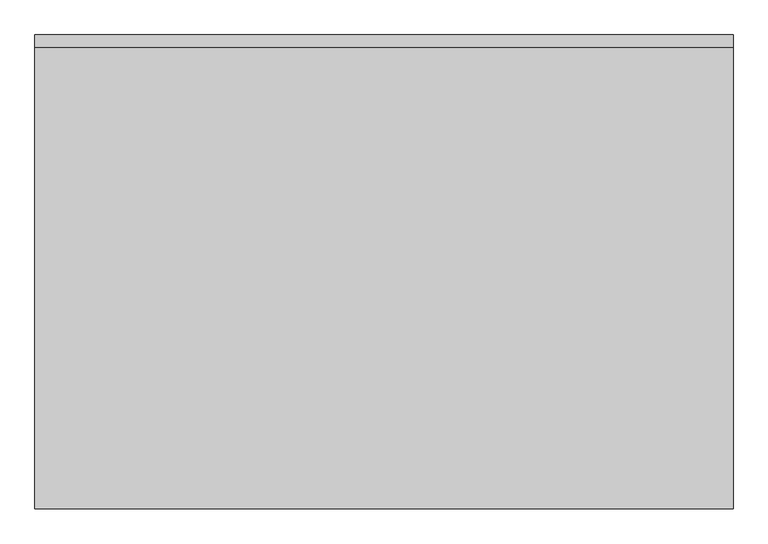
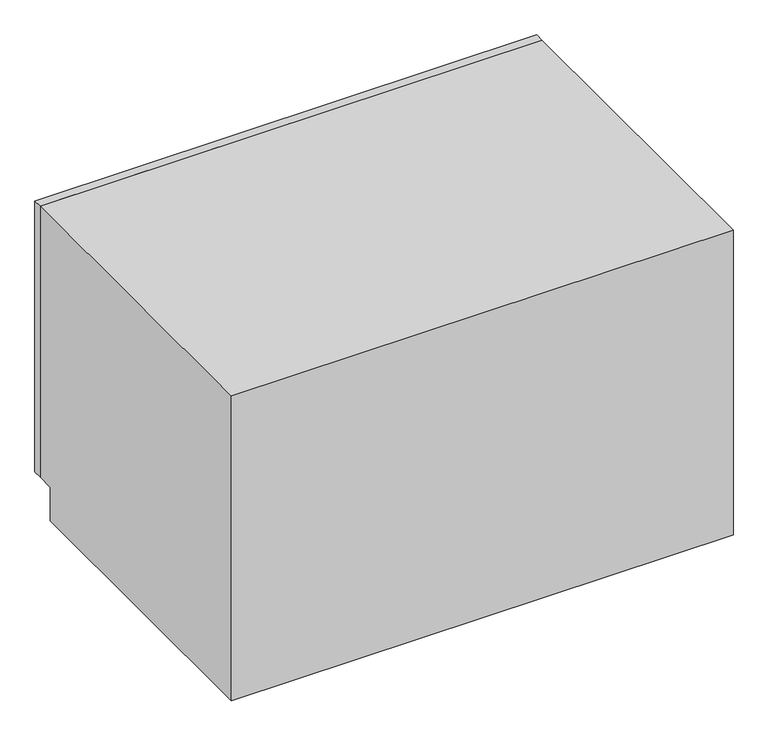
"""IFC4 building model written with IfcOpenShell, lengths in millimetres: furniture geometry, OD_CW_Base Cabinet : OD_CW_Base Cabinet."""

from ifc_helpers import new_model, si_unit, frame, origin, place, context, project, spatial, polyline, outline, extrude, source, transform, mapped, element, save


def furniture_dfc94ca7(model_context):
    return source(origin(), model_context, "Body", "SweptSolid", [
        extrude(outline(polyline([(18.7377049, 330.2), (18.7377049, 355.6), (1441.1377049, 355.6), (1441.1377049, 330.2), (18.7377049, 330.2)])), frame((0.0, 0.0, 101.6), z_axis=(0.0, 0.0, 1.0), x_axis=(1.0, 0.0, 0.0)), (0.0, 0.0, 1.0), 812.8),
        extrude(outline(polyline([(330.2, 914.4), (330.2, 101.6), (279.4, 101.6), (279.4, 0.0), (-609.6, 0.0), (-609.6, 914.4), (330.2, 914.4)])), frame((18.7377049, 0.0, 0.0), z_axis=(1.0, 0.0, 0.0), x_axis=(0.0, 1.0, 0.0)), (0.0, 0.0, 1.0), 1422.4),
    ])


if __name__ == "__main__":
    model = new_model("IFC4")
    model_context = context("Model", 3, world=origin())
    ifc_project = project(units=[si_unit("LENGTHUNIT", "METRE", prefix="MILLI")], contexts=[model_context])
    site = spatial("IfcSite", under=ifc_project)
    building = spatial("IfcBuilding", under=site)
    placement = place(None, origin())
    furniture_shape = furniture_dfc94ca7(model_context)
    element("IfcFurniture", 1, ObjectType="OD_CW_Base Cabinet : OD_CW_Base Cabinet", at=placement, inside=building, context=model_context, shape_type="MappedRepresentation", body=[
        mapped(furniture_shape, transform((0.0, 0.0, 0.0), x_axis=(1.0, 0.0, 0.0), y_axis=(0.0, 1.0, 0.0), z_axis=(0.0, 0.0, 1.0))),
    ])
    save(model, "model.ifc")

# Revit data of these elements
# Type "OD_CW_Base Cabinet : OD_CW_Base Cabinet"
#   OD_CW_Width [instance default] = 2' - 10"
#   OD_CW_Length [instance default] = 8' - 0"
#   OD_CW_Height [instance default] = 2' - 3"
#   Depth = 2' - 0"
#   Height = 3' - 0"
#   Width = 4' - 0"
#   OD_CW_Material_Front Panel [instance default] = none
#   OD_CW_Material_Body [instance default] = none
# Element 1 (IfcFurniture, "OD_CW_Base Cabinet : OD_CW_Base Cabinet")
#   OD_CW_Width = 3' - 2"
#   OD_CW_Length = 4' - 8"
#   OD_CW_Height = 3' - 0"
#   OD_CW_Material_Body = DISH CLEAN TABLE
#   Materials on its faces: "DISH CLEAN TABLE", "CASEWORK"
# Materials
#   "DISH CLEAN TABLE": class "Generic", colour RGB 187 187 187, transparency 0, Cost = 0
#   "CASEWORK": class "Generic", colour RGB 181 181 181, transparency 0, Cost = 0
